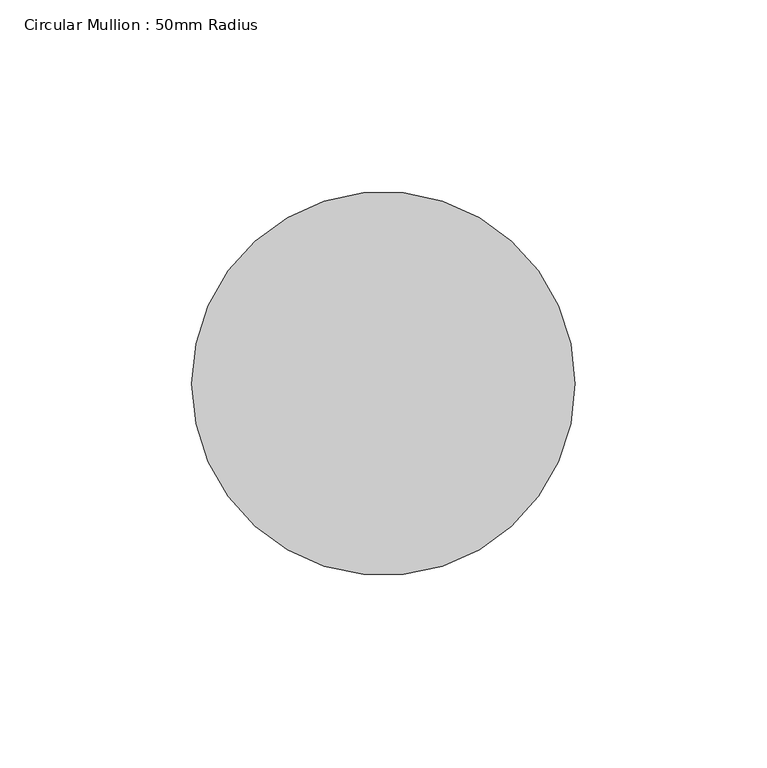
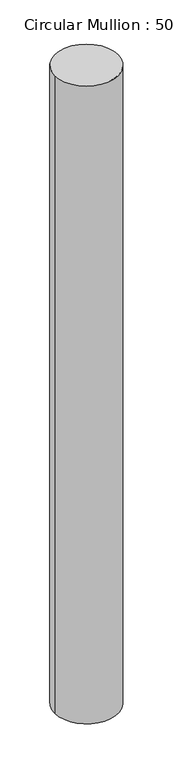
"""IFC4 building model written with IfcOpenShell, lengths in millimetres: member geometry, Circular Mullion : 50mm Radius."""

from ifc_helpers import new_model, si_unit, point, frame, origin, origin_2d, place, context, project, spatial, circle_curve, trimmed, segment, composite_curve, outline, extrude, source, transform, mapped, element, save


def circular_mullion_50mm_radius_a0d2f8bc(model_context):
    return source(origin(), model_context, "Body", "SweptSolid", [
        extrude(outline(composite_curve([segment(trimmed(circle_curve(origin_2d(), 50.0), [point((50.0, 0.0))], [point((-50.0, 0.0))], False, "CARTESIAN"), True, "CONTINUOUS"), segment(trimmed(circle_curve(origin_2d(), 50.0), [point((-50.0, 0.0))], [point((50.0, 0.0))], False, "CARTESIAN"), True, "CONTINUOUS")], self_intersect=False)), frame((0.0, 0.0, -1066.199131), z_axis=(0.0, 0.0, 1.0), x_axis=(1.0, 0.0, 0.0)), (0.0, 0.0, 1.0), 1066.199131),
    ])


if __name__ == "__main__":
    model = new_model("IFC4")
    model_context = context("Model", 3, world=origin())
    ifc_project = project(units=[si_unit("LENGTHUNIT", "METRE", prefix="MILLI")], contexts=[model_context])
    site = spatial("IfcSite", under=ifc_project)
    building = spatial("IfcBuilding", under=site)
    placement = place(None, origin())
    circular_mullion_50mm_radius_shape = circular_mullion_50mm_radius_a0d2f8bc(model_context)
    element("IfcMember", 1, ObjectType="Circular Mullion : 50mm Radius", at=placement, inside=building, context=model_context, shape_type="MappedRepresentation", body=[
        mapped(circular_mullion_50mm_radius_shape, transform((0.0, 0.0, 0.0), x_axis=(1.0, 0.0, 0.0), y_axis=(0.0, 1.0, 0.0), z_axis=(0.0, 0.0, 1.0))),
    ])
    save(model, "model.ifc")

# Revit data of these elements
# Type "Circular Mullion : 50mm Radius"
#   built-in parameter 1007350 = 0.164042 (stored number, unit not read)
# Element 1 (IfcMember, "Circular Mullion : 50mm Radius")
#   Materials on its faces: "Aluminium"
# Materials
#   "Aluminium": class "Metal", colour RGB 247 247 247, transparency 0, Description = "Aluminium 6061", Cost = 0
